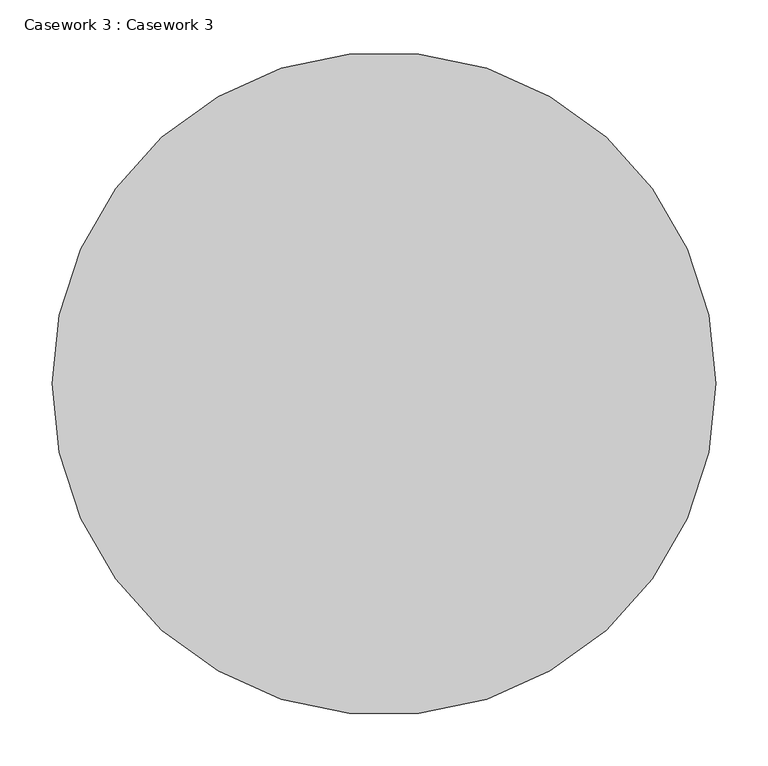
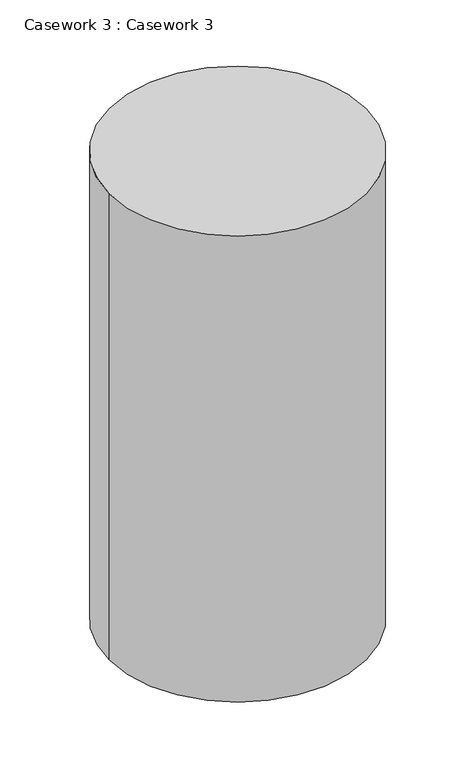
"""IFC4 building model written with IfcOpenShell, lengths in millimetres: furniture geometry, Casework 3 : Casework 3."""

from ifc_helpers import new_model, si_unit, point, frame_2d, origin, origin_with_axes, place, context, project, spatial, circle_curve, trimmed, segment, composite_curve, outline, extrude, source, transform, mapped, element, save


def casework_3_casework_3_f1c2039d(model_context):
    return source(origin(), model_context, "Body", "SweptSolid", [
        extrude(outline(composite_curve([segment(trimmed(circle_curve(frame_2d((-40793.717289, 250978.0781331)), 317.826855), [point((-41111.544144, 250978.0781331))], [point((-40475.8904339, 250978.0781331))], False, "CARTESIAN"), True, "CONTINUOUS"), segment(trimmed(circle_curve(frame_2d((-40793.717289, 250978.0781331)), 317.826855), [point((-40475.8904339, 250978.0781331))], [point((-41111.544144, 250978.0781331))], False, "CARTESIAN"), True, "CONTINUOUS")], self_intersect=False)), origin_with_axes(), (0.0, 0.0, 1.0), 1219.2),
    ])


if __name__ == "__main__":
    model = new_model("IFC4")
    model_context = context("Model", 3, world=origin())
    ifc_project = project(units=[si_unit("LENGTHUNIT", "METRE", prefix="MILLI")], contexts=[model_context])
    site = spatial("IfcSite", under=ifc_project)
    building = spatial("IfcBuilding", under=site)
    placement = place(None, origin())
    casework_3_casework_3_shape = casework_3_casework_3_f1c2039d(model_context)
    element("IfcFurniture", 1, ObjectType="Casework 3 : Casework 3", at=placement, inside=building, context=model_context, shape_type="MappedRepresentation", body=[
        mapped(casework_3_casework_3_shape, transform((0.0, 0.0, 0.0), x_axis=(1.0, 0.0, 0.0), y_axis=(0.0, 1.0, 0.0), z_axis=(0.0, 0.0, 1.0))),
    ])
    save(model, "model.ifc")

# Revit data of these elements
# Element 1 (IfcFurniture, "Casework 3 : Casework 3")
#   Materials on its faces: "DOUGH MIXER"
# Materials
#   "DOUGH MIXER": class "Generic", colour RGB 187 187 187, transparency 0, Cost = 0
